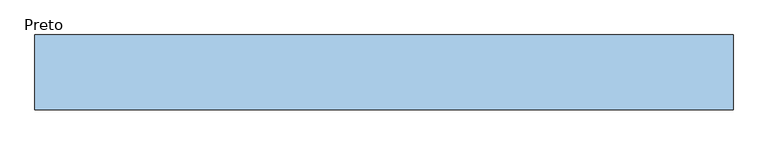
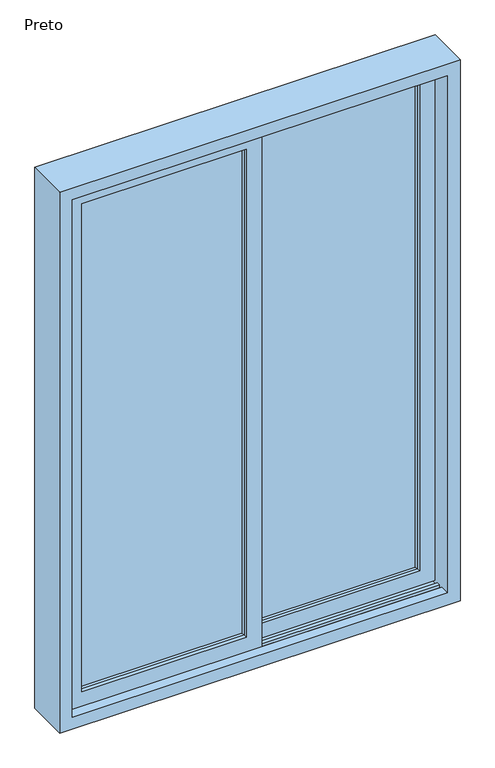
"""IFC4 building model written with IfcOpenShell, lengths in millimetres: window geometry, Blks_Cons Weiku_Janela de Correr 02 Folhas : Preto."""

from ifc_helpers import new_model, si_unit, frame, origin, place, context, project, spatial, polyline, outline, extrude, faceted_brep, source, transform, mapped, element, save


def preto_a1bd591b(model_context):
    return source(origin(), model_context, "Body", "SolidModel", [
        faceted_brep([(27.0, 13.0, 898.0), (27.0, 13.0, 2702.0), (27.0, 18.0, 2702.0), (27.0, 18.0, 898.0), (32.0, 18.0, 903.0), (32.0, 18.0, 2697.0), (602.0, 13.0, 2702.0), (602.0, 18.0, 2702.0), (597.0, 18.0, 2697.0), (602.0, 13.0, 898.0), (602.0, 18.0, 898.0), (597.0, 18.0, 903.0)], [[[0, 1, 2, 3]], [[4, 5, 1, 0]], [[1, 6, 7, 2]], [[5, 8, 6, 1]], [[6, 9, 10, 7]], [[8, 11, 9, 6]], [[3, 2, 7, 10], [5, 4, 11, 8]], [[9, 0, 3, 10]], [[11, 4, 0, 9]]]),
        faceted_brep([(602.0, 27.0, 898.0), (602.0, 27.0, 2702.0), (602.0, 22.0, 2702.0), (602.0, 22.0, 898.0), (27.0, 27.0, 2702.0), (27.0, 22.0, 2702.0), (27.0, 27.0, 898.0), (27.0, 22.0, 898.0), (597.0, 22.0, 2697.0), (597.0, 22.0, 903.0), (32.0, 22.0, 903.0), (32.0, 22.0, 2697.0)], [[[0, 1, 2, 3]], [[1, 4, 5, 2]], [[4, 6, 7, 5]], [[3, 2, 5, 7], [8, 9, 10, 11]], [[6, 0, 3, 7]], [[9, 8, 1, 0]], [[8, 11, 4, 1]], [[11, 10, 6, 4]], [[10, 9, 0, 6]]]),
        extrude(outline(polyline([(602.0, 22.0), (602.0, 18.0), (27.0, 18.0), (27.0, 22.0), (602.0, 22.0)])), frame((0.0, 0.0, 898.0), z_axis=(0.0, 0.0, 1.0), x_axis=(1.0, 0.0, 0.0)), (0.0, 0.0, 1.0), 1804.0),
        extrude(outline(polyline([(844.0, 656.0), (2756.0, 656.0), (2756.0, -27.0), (844.0, -27.0), (844.0, 656.0)]), holes=[polyline([(2702.0, 27.0), (2702.0, 602.0), (898.0, 602.0), (898.0, 27.0), (2702.0, 27.0)])]), frame((0.0, 0.0, 0.0), z_axis=(0.0, 1.0, 0.0), x_axis=(0.0, 0.0, 1.0)), (0.0, 0.0, 1.0), 40.0),
        faceted_brep([(-602.0, -27.0, 898.0), (-602.0, -27.0, 2702.0), (-602.0, -22.0, 2702.0), (-602.0, -22.0, 898.0), (-597.0, -22.0, 903.0), (-597.0, -22.0, 2697.0), (-27.0, -27.0, 2702.0), (-27.0, -22.0, 2702.0), (-32.0, -22.0, 2697.0), (-27.0, -27.0, 898.0), (-27.0, -22.0, 898.0), (-32.0, -22.0, 903.0)], [[[0, 1, 2, 3]], [[4, 5, 1, 0]], [[1, 6, 7, 2]], [[5, 8, 6, 1]], [[6, 9, 10, 7]], [[8, 11, 9, 6]], [[3, 2, 7, 10], [5, 4, 11, 8]], [[9, 0, 3, 10]], [[11, 4, 0, 9]]]),
        faceted_brep([(-27.0, -13.0, 898.0), (-27.0, -13.0, 2702.0), (-27.0, -18.0, 2702.0), (-27.0, -18.0, 898.0), (-602.0, -13.0, 2702.0), (-602.0, -18.0, 2702.0), (-602.0, -13.0, 898.0), (-602.0, -18.0, 898.0), (-32.0, -18.0, 2697.0), (-32.0, -18.0, 903.0), (-597.0, -18.0, 903.0), (-597.0, -18.0, 2697.0)], [[[0, 1, 2, 3]], [[1, 4, 5, 2]], [[4, 6, 7, 5]], [[3, 2, 5, 7], [8, 9, 10, 11]], [[6, 0, 3, 7]], [[9, 8, 1, 0]], [[8, 11, 4, 1]], [[11, 10, 6, 4]], [[10, 9, 0, 6]]]),
        extrude(outline(polyline([(-27.0, -18.0), (-27.0, -22.0), (-602.0, -22.0), (-602.0, -18.0), (-27.0, -18.0)])), frame((0.0, 0.0, 898.0), z_axis=(0.0, 0.0, 1.0), x_axis=(1.0, 0.0, 0.0)), (0.0, 0.0, 1.0), 1804.0),
        extrude(outline(polyline([(844.0, 27.0), (2756.0, 27.0), (2756.0, -656.0), (844.0, -656.0), (844.0, 27.0)]), holes=[polyline([(2702.0, -602.0), (2702.0, -27.0), (898.0, -27.0), (898.0, -602.0), (2702.0, -602.0)])]), frame((0.0, -40.0, 0.0), z_axis=(0.0, 1.0, 0.0), x_axis=(0.0, 0.0, 1.0)), (0.0, 0.0, 1.0), 40.0),
        faceted_brep([(656.0, -75.0, 844.0), (656.0, -40.0, 844.0), (-656.0, -40.0, 844.0), (-656.0, -75.0, 844.0), (-656.0, 75.0, 844.0), (-656.0, 40.0, 844.0), (656.0, 40.0, 844.0), (656.0, 75.0, 844.0), (-656.0, 13.0, 844.0), (656.0, 13.0, 844.0), (656.0, 27.0, 844.0), (-656.0, 27.0, 844.0), (-656.0, -27.0, 844.0), (656.0, -27.0, 844.0), (656.0, -13.0, 844.0), (-656.0, -13.0, 844.0), (700.0, -75.0, 800.0), (700.0, -75.0, 2800.0), (-700.0, -75.0, 2800.0), (-700.0, -75.0, 800.0), (-656.0, -75.0, 2756.0), (656.0, -75.0, 2756.0), (-656.0, -40.0, 834.0), (-656.0, -27.0, 834.0), (-656.0, -13.0, 834.0), (-656.0, 13.0, 834.0), (-656.0, 27.0, 834.0), (-656.0, 40.0, 834.0), (-656.0, 75.0, 2756.0), (-656.0, 40.0, 2756.0), (-656.0, 40.0, 2766.0), (-656.0, 27.0, 2766.0), (-656.0, 27.0, 2756.0), (-656.0, 13.0, 2756.0), (-656.0, 13.0, 2766.0), (-656.0, -13.0, 2766.0), (-656.0, -13.0, 2756.0), (-656.0, -27.0, 2756.0), (-656.0, -27.0, 2766.0), (-656.0, -40.0, 2766.0), (-656.0, -40.0, 2756.0), (656.0, -40.0, 834.0), (656.0, -40.0, 2756.0), (656.0, -40.0, 2766.0), (656.0, -27.0, 2766.0), (656.0, -27.0, 2756.0), (656.0, -13.0, 2756.0), (656.0, -13.0, 2766.0), (656.0, 13.0, 2766.0), (656.0, 13.0, 2756.0), (656.0, 27.0, 2756.0), (656.0, 27.0, 2766.0), (656.0, 40.0, 2766.0), (656.0, 40.0, 2756.0), (656.0, 75.0, 2756.0), (656.0, 40.0, 834.0), (656.0, 27.0, 834.0), (656.0, 13.0, 834.0), (656.0, -13.0, 834.0), (656.0, -27.0, 834.0), (-700.0, 75.0, 800.0), (-700.0, 75.0, 2800.0), (700.0, 75.0, 2800.0), (700.0, 75.0, 800.0)], [[[0, 1, 2, 3]], [[4, 5, 6, 7]], [[8, 9, 10, 11]], [[12, 13, 14, 15]], [[16, 17, 18, 19], [3, 20, 21, 0]], [[3, 2, 22, 23, 12, 15, 24, 25, 8, 11, 26, 27, 5, 4, 28, 29, 30, 31, 32, 33, 34, 35, 36, 37, 38, 39, 40, 20]], [[22, 2, 1, 41]], [[21, 42, 43, 44, 45, 46, 47, 48, 49, 50, 51, 52, 53, 54, 7, 6, 55, 56, 10, 9, 57, 58, 14, 13, 59, 41, 1, 0]], [[60, 61, 62, 63], [7, 54, 28, 4]], [[55, 6, 5, 27]], [[56, 26, 11, 10]], [[9, 8, 25, 57]], [[58, 24, 15, 14]], [[13, 12, 23, 59]], [[63, 62, 17, 16]], [[16, 19, 60, 63]], [[19, 18, 61, 60]], [[55, 27, 26, 56]], [[57, 25, 24, 58]], [[59, 23, 22, 41]], [[20, 40, 42, 21]], [[54, 53, 29, 28]], [[32, 50, 49, 33]], [[36, 46, 45, 37]], [[18, 17, 62, 61]], [[46, 36, 35, 47]], [[47, 35, 34, 48]], [[48, 34, 33, 49]], [[50, 32, 31, 51]], [[51, 31, 30, 52]], [[30, 29, 53, 52]], [[43, 42, 40, 39]], [[43, 39, 38, 44]], [[44, 38, 37, 45]]]),
    ])


if __name__ == "__main__":
    model = new_model("IFC4")
    model_context = context("Model", 3, world=origin())
    ifc_project = project(units=[si_unit("LENGTHUNIT", "METRE", prefix="MILLI")], contexts=[model_context])
    site = spatial("IfcSite", under=ifc_project)
    building = spatial("IfcBuilding", under=site)
    placement = place(None, origin())
    preto_shape = preto_a1bd591b(model_context)
    element("IfcWindow", 1, ObjectType="Blks_Cons Weiku_Janela de Correr 02 Folhas : Preto", at=placement, inside=building, context=model_context, shape_type="MappedRepresentation", body=[
        mapped(preto_shape, transform((0.0, 0.0, 0.0), x_axis=(1.0, 0.0, 0.0), y_axis=(0.0, 1.0, 0.0), z_axis=(0.0, 0.0, 1.0))),
    ])
    save(model, "model.ifc")

# Revit data of these elements
# Type "Blks_Cons Weiku_Janela de Correr 02 Folhas : Preto"
#   Type Mark = "J26"
#   Type Comments = "Janela de Correr 02 Folhas"
#   Manufacturer = "Weiku"
#   Created By / Criado Por / Creado por = "Blocks"
#   Author URL = "https://BlocksRvt.com/"
#   Author Contact = "info@blocksrvt.com"
#   Assembly Code = "Cons"
#   c [instance default] = 250 mm
#   b [instance default] = 912 mm
#   a [instance default] = 983 mm
#   Rough Width [instance default] = 2000 mm
#   Width [instance default] = 1912 mm
#   Espessura Folha [instance default] = 40 mm
#   Rough Height [instance default] = 1000 mm
#   Height [instance default] = 912 mm
#   Abertura Janela Equerda [instance default] = 0 mm
#   Abertura Janela Direita [instance default] = 0 mm
#   Vidro = .vidro_growarq
#   Vedação = Blks - Rubber - Black
#   Janela = Blks - Plastic - Black - Glazed
#   Wall Closure = (empty or 0)
# Element 1 (IfcWindow, "Blks_Cons Weiku_Janela de Correr 02 Folhas : Preto")
#   b = 1912 mm
#   a = 683 mm
#   Rough Width = 1400 mm
#   Width = 1312 mm
#   Rough Height = 2000 mm
#   Height = 1912 mm
#   Materials on its faces: "Blks - Plastic - Black - Glazed", "Blks - Rubber - Black", ".vidro_growarq"
# Materials
#   ".vidro_growarq": class "Vidro", colour RGB 200 215 215, transparency 0.6, Description = "Vidroverde", Cost = 0
#   "Blks - Rubber - Black": class "Paint/Coating", colour RGB 38 38 38, transparency 0, Cost = 0
#   "Blks - Plastic - Black - Glazed": class "Plastic", colour RGB 25 25 25, transparency 0, Cost = 0
